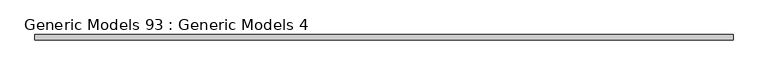
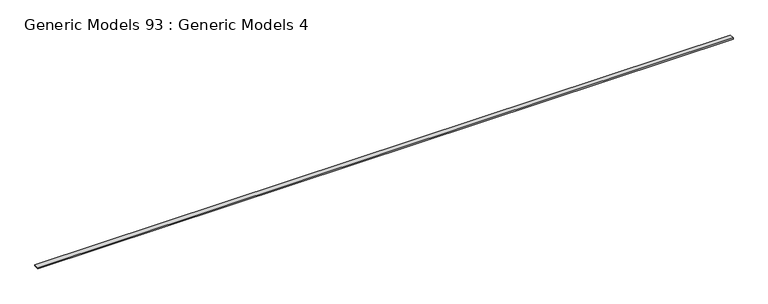
"""IFC4 building model written with IfcOpenShell, lengths in millimetres: proxy geometry, Generic Models 93 : Generic Models 4."""

from ifc_helpers import new_model, si_unit, frame, origin, place, context, project, spatial, polyline, outline, extrude, source, transform, mapped, element, save


def generic_models_93_generic_models_4_01b8dabe(model_context):
    return source(origin(), model_context, "Body", "SweptSolid", [
        extrude(outline(polyline([(51294.7476718, 127104.4735933), (51294.7476718, 127142.5735933), (51434.4476718, 127136.7527599), (51434.4476718, 127104.4735933), (51294.7476718, 127104.4735933)])), frame((-20795.7733045, 0.0, 0.0), z_axis=(1.0, 0.0, 0.0), x_axis=(0.0, 1.0, 0.0)), (0.0, 0.0, 1.0), 18643.6),
    ])


if __name__ == "__main__":
    model = new_model("IFC4")
    model_context = context("Model", 3, world=origin())
    ifc_project = project(units=[si_unit("LENGTHUNIT", "METRE", prefix="MILLI")], contexts=[model_context])
    site = spatial("IfcSite", under=ifc_project)
    building = spatial("IfcBuilding", under=site)
    placement = place(None, origin())
    generic_models_93_generic_models_4_shape = generic_models_93_generic_models_4_01b8dabe(model_context)
    element("IfcBuildingElementProxy", 1, Name="Generic Models 93 : Generic Models 4", ObjectType="Generic Models 93 : Generic Models 4", at=placement, inside=building, context=model_context, shape_type="MappedRepresentation", body=[
        mapped(generic_models_93_generic_models_4_shape, transform((0.0, 0.0, 0.0), x_axis=(1.0, 0.0, 0.0), y_axis=(0.0, 1.0, 0.0), z_axis=(0.0, 0.0, 1.0))),
    ])
    save(model, "model.ifc")

# Revit data of these elements
# Element 1 (IfcBuildingElementProxy, "Generic Models 93 : Generic Models 4")
#   Materials on its faces: "_2X BLOCKING AS REQUIRED"
# Materials
#   "_2X BLOCKING AS REQUIRED": class "Generic", colour RGB 177 130 114, transparency 0, Cost = 0
